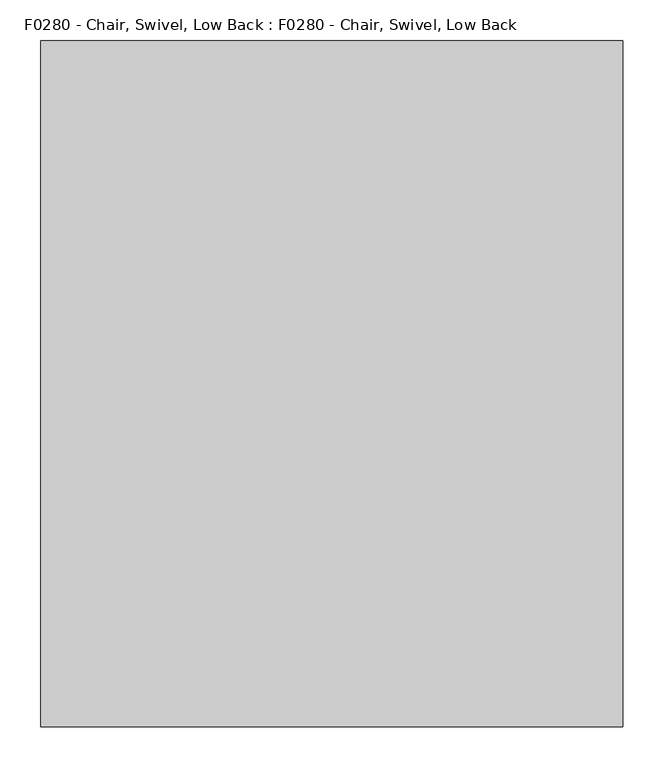
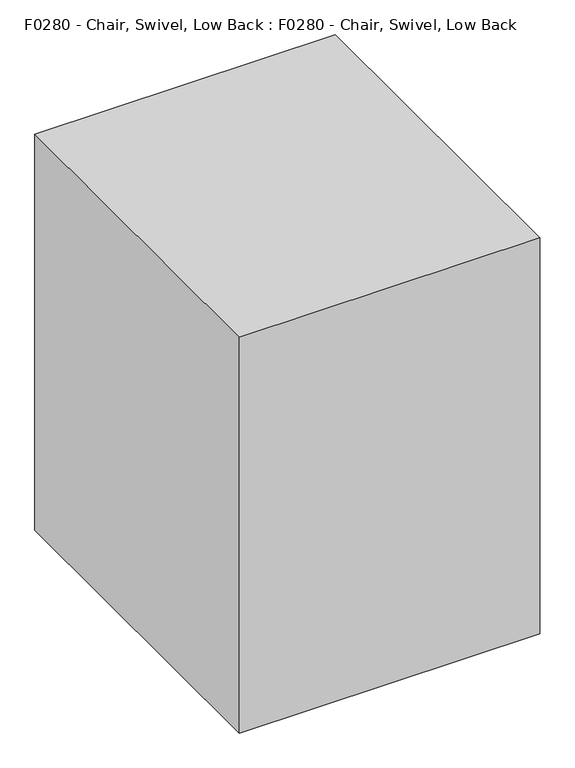
"""IFC4 building model written with IfcOpenShell, lengths in millimetres: proxy geometry, F0280 - Chair, Swivel, Low Back : F0280 - Chair, Swivel, Low Back."""

import ifcopenshell
import ifcopenshell.guid

model = None  # the IFC model being written
_history = None  # IfcOwnerHistory: only IFC2X3 demands one
_inside = {}  # id of a spatial element -> (the spatial element, [elements in it])
_under = {}  # id of a project, library or spatial element -> (it, [spatial elements below it])
_declared = {}  # id of a project -> (the project, [libraries it declares])
_typed = {}  # id of a type object -> (the type object, [elements of that type])
_made_of = {}  # id of a material, layer set ... -> (it, [elements and type objects made of it])


def new_model(schema):
    """Start an empty IFC model of exactly this schema.

    Asked for "IFC4X3", IfcOpenShell would pick the latest addendum, in which some entities
    have other attributes; the version numbers below select the first issue.
    IFC2X3 requires an IfcOwnerHistory on every rooted entity: one is made here for all.
    """
    global model, _history
    if schema == "IFC4X3":
        model = ifcopenshell.file(schema_version=(4, 3, 0, 0))
    else:
        model = ifcopenshell.file(schema=schema)
    _inside.clear()
    _under.clear()
    _declared.clear()
    _typed.clear()
    _made_of.clear()
    _history = None
    if model.schema == "IFC2X3":
        org = make("IfcOrganization", Name="unknown")
        user = make(
            "IfcPersonAndOrganization",
            ThePerson=make("IfcPerson", FamilyName="unknown"),
            TheOrganization=org,
        )
        app = make(
            "IfcApplication",
            ApplicationDeveloper=org,
            Version="unknown",
            ApplicationFullName="unknown",
            ApplicationIdentifier="unknown",
        )
        _history = make(
            "IfcOwnerHistory",
            OwningUser=user,
            OwningApplication=app,
            ChangeAction="ADDED",
            CreationDate=0,
        )
    return model


def make(cls, **values):
    """One entity of the class cls with the attributes given. An attribute that is None is left unset."""
    return model.create_entity(
        cls, **{name: value for name, value in values.items() if value is not None}
    )


def rooted(cls, **values):
    """An entity with a GlobalId (a new one), such as an element, a storey or a relation."""
    return make(cls, GlobalId=ifcopenshell.guid.new(), OwnerHistory=_history, **values)


def si_unit(unit_type, name, prefix=None):
    """IfcSIUnit, for example si_unit("LENGTHUNIT", "METRE", prefix="MILLI")."""
    return make("IfcSIUnit", UnitType=unit_type, Prefix=prefix, Name=name)


def assignment(units):
    """IfcUnitAssignment: the units of a project."""
    return None if units is None else make("IfcUnitAssignment", Units=units)


def point(xyz):
    """IfcCartesianPoint."""
    return None if xyz is None else make("IfcCartesianPoint", Coordinates=xyz)


def direction(xyz):
    """IfcDirection."""
    return None if xyz is None else make("IfcDirection", DirectionRatios=xyz)


def frame(location, z_axis=None, x_axis=None):
    """IfcAxis2Placement3D, a coordinate frame: its origin and axes. An axis left out is left unset."""
    return make(
        "IfcAxis2Placement3D",
        Location=point(location),
        Axis=direction(z_axis),
        RefDirection=direction(x_axis),
    )


def frame_2d(location, x_axis=None):
    """IfcAxis2Placement2D, a coordinate frame in the plane: its origin and x axis."""
    return make(
        "IfcAxis2Placement2D", Location=point(location), RefDirection=direction(x_axis)
    )


def origin():
    """The frame at (0, 0, 0) with its axes left unset."""
    return frame((0.0, 0.0, 0.0))


def origin_with_axes():
    """The frame at (0, 0, 0) with the z axis (0, 0, 1) and the x axis (1, 0, 0) written out."""
    return frame((0.0, 0.0, 0.0), z_axis=(0.0, 0.0, 1.0), x_axis=(1.0, 0.0, 0.0))


def origin_2d():
    """The frame at (0, 0) in the plane with its x axis left unset."""
    return frame_2d((0.0, 0.0))


def place(relative_to, where):
    """IfcLocalPlacement: puts the frame where relative to a parent placement (None: the world)."""
    return make(
        "IfcLocalPlacement", PlacementRelTo=relative_to, RelativePlacement=where
    )


def context(
    kind, dimensions, precision=None, world=None, true_north=None, identifier=None
):
    """IfcGeometricRepresentationContext, for example the 3D "Model" context."""
    return make(
        "IfcGeometricRepresentationContext",
        ContextIdentifier=identifier,
        ContextType=kind,
        CoordinateSpaceDimension=dimensions,
        Precision=precision,
        WorldCoordinateSystem=world,
        TrueNorth=true_north,
    )


def project(units=None, contexts=None):
    """IfcProject with its units and contexts."""
    return rooted(
        "IfcProject",
        Name="project",
        RepresentationContexts=contexts,
        UnitsInContext=assignment(units),
    )


def spatial(cls, under=None, at=None, **own):
    """A site, building, storey or space (cls), placed at a placement, below another one or the project."""
    s = rooted(cls, ObjectPlacement=at, **own)
    if under is not None:
        _under.setdefault(under.id(), (under, []))[1].append(s)
    return s


def polyline(points):
    """IfcPolyline through the points."""
    return make("IfcPolyline", Points=[point(p) for p in points])


def circle_curve(where, radius):
    """IfcCircle in the frame where."""
    return make("IfcCircle", Position=where, Radius=radius)


def ellipse_curve(where, semi_axis1, semi_axis2):
    """IfcEllipse in the frame where."""
    return make(
        "IfcEllipse", Position=where, SemiAxis1=semi_axis1, SemiAxis2=semi_axis2
    )


def trimmed(basis, trim1, trim2, sense, master):
    """IfcTrimmedCurve: the piece of a basis curve between two trims."""
    return make(
        "IfcTrimmedCurve",
        BasisCurve=basis,
        Trim1=trim1,
        Trim2=trim2,
        SenseAgreement=sense,
        MasterRepresentation=master,
    )


def segment(curve, same_sense, transition):
    """IfcCompositeCurveSegment."""
    return make(
        "IfcCompositeCurveSegment",
        Transition=transition,
        SameSense=same_sense,
        ParentCurve=curve,
    )


def composite_curve(segments, self_intersect=None):
    """IfcCompositeCurve: segments joined end to end."""
    return make("IfcCompositeCurve", Segments=segments, SelfIntersect=self_intersect)


def outline(outer, holes=None, kind="AREA"):
    """IfcArbitraryClosedProfileDef: a profile drawn as a closed curve; with holes, ...WithVoids."""
    if holes is None:
        return make("IfcArbitraryClosedProfileDef", ProfileType=kind, OuterCurve=outer)
    return make(
        "IfcArbitraryProfileDefWithVoids",
        ProfileType=kind,
        OuterCurve=outer,
        InnerCurves=holes,
    )


def extrude(swept, where, along, depth):
    """IfcExtrudedAreaSolid: the profile swept, set in the frame where, extruded along a direction by depth."""
    return make(
        "IfcExtrudedAreaSolid",
        SweptArea=swept,
        Position=where,
        ExtrudedDirection=direction(along),
        Depth=depth,
    )


def shape(context_of_items, identifier, shape_type, items):
    """IfcShapeRepresentation: the items that make up one representation, for example the "Body"."""
    return make(
        "IfcShapeRepresentation",
        ContextOfItems=context_of_items,
        RepresentationIdentifier=identifier,
        RepresentationType=shape_type,
        Items=items,
    )


def source(mapping_origin, context_of_items, identifier, shape_type, items):
    """IfcRepresentationMap: a shape defined once, which mapped items show again and again."""
    return make(
        "IfcRepresentationMap",
        MappingOrigin=mapping_origin,
        MappedRepresentation=shape(context_of_items, identifier, shape_type, items),
    )


def transform(
    local_origin,
    x_axis=None,
    y_axis=None,
    z_axis=None,
    scale=None,
    scale2=None,
    scale3=None,
    uniform=True,
):
    """IfcCartesianTransformationOperator3D, or its non-uniform kind. x_axis, y_axis, z_axis: its Axis1, 2, 3."""
    if uniform:
        return make(
            "IfcCartesianTransformationOperator3D",
            Axis1=direction(x_axis),
            Axis2=direction(y_axis),
            LocalOrigin=point(local_origin),
            Scale=scale,
            Axis3=direction(z_axis),
        )
    return make(
        "IfcCartesianTransformationOperator3DnonUniform",
        Axis1=direction(x_axis),
        Axis2=direction(y_axis),
        LocalOrigin=point(local_origin),
        Scale=scale,
        Axis3=direction(z_axis),
        Scale2=scale2,
        Scale3=scale3,
    )


def mapped(mapping_source, mapping_target):
    """IfcMappedItem: shows the shape of a source again, moved by a transform."""
    return make(
        "IfcMappedItem", MappingSource=mapping_source, MappingTarget=mapping_target
    )


def made_of(thing, what):
    """Note that an element or type object is made of a material, layer set ...; save() writes the relation."""
    if what is not None:
        _made_of.setdefault(what.id(), (what, []))[1].append(thing)
    return thing


def element(
    cls,
    number,
    at=None,
    inside=None,
    cuts=None,
    type_object=None,
    material=None,
    context=None,
    identifier="Body",
    shape_type=None,
    held_by="IfcProductDefinitionShape",
    body=None,
    shapes=None,
    **own,
):
    """One element of the class cls, such as IfcWall. Its Tag is "e" and its number.

    at: its placement. inside: the storey or other place that contains it. cuts: it is an
    opening in that element (IfcRelVoidsElement). A single representation is given by context,
    identifier, shape_type and body (its items); several are given by shapes. held_by: the class
    of the entity that holds the representations. save() writes the other relations.
    """
    e = rooted(cls, Tag="e%d" % number, ObjectPlacement=at, **own)
    if body is not None:
        shapes = [shape(context, identifier, shape_type, body)]
    if shapes is not None:
        e.Representation = make(held_by, Representations=shapes)
    if inside is not None:
        _inside.setdefault(inside.id(), (inside, []))[1].append(e)
    if cuts is not None:
        rooted(
            "IfcRelVoidsElement", RelatingBuildingElement=cuts, RelatedOpeningElement=e
        )
    if type_object is not None:
        _typed.setdefault(type_object.id(), (type_object, []))[1].append(e)
    return made_of(e, material)


def aggregate(whole, parts):
    """IfcRelAggregates: a whole, such as a stair, and the parts it consists of."""
    return rooted("IfcRelAggregates", RelatingObject=whole, RelatedObjects=parts)


def save(model, path):
    """Write the relations noted so far, then the file.

    IfcRelAggregates (storeys below a building ...), IfcRelContainedInSpatialStructure (elements
    in a storey), IfcRelDefinesByType, IfcRelAssociatesMaterial and IfcRelDeclares: one each for
    every whole, place, type object, material and project.
    """
    for whole, parts in _under.values():
        aggregate(whole, parts)
    for where, things in _inside.values():
        rooted(
            "IfcRelContainedInSpatialStructure",
            RelatedElements=things,
            RelatingStructure=where,
        )
    for kind, things in _typed.values():
        rooted("IfcRelDefinesByType", RelatedObjects=things, RelatingType=kind)
    for what, things in _made_of.values():
        rooted("IfcRelAssociatesMaterial", RelatedObjects=things, RelatingMaterial=what)
    for by, libraries in _declared.values():
        rooted("IfcRelDeclares", RelatingContext=by, RelatedDefinitions=libraries)
    model.write(path)


def plane_surface(at):
    """IfcPlane: the flat surface through the origin of the frame at, square to its z axis."""
    return make("IfcPlane", Position=at)


def cylinder_surface(at, radius):
    """IfcCylindricalSurface: all points at the distance radius from the z axis of the frame at."""
    return make("IfcCylindricalSurface", Position=at, Radius=radius)


def revolved_surface(curve, axis_point, axis_direction):
    """IfcSurfaceOfRevolution: the curve turned about the line through axis_point along axis_direction."""
    return make(
        "IfcSurfaceOfRevolution",
        SweptCurve=make("IfcArbitraryOpenProfileDef", ProfileType="CURVE", Curve=curve),
        AxisPosition=make("IfcAxis1Placement", Location=point(axis_point), Axis=direction(axis_direction)),
    )


def advanced_brep(points, edges, surfaces, faces):
    """IfcAdvancedBrep: a solid bounded by faces that lie on surfaces and meet in shared edges.

    An edge is (start, end): straight between two places in points (the first is 0);
    or (start, end, curve); or (start, end, curve, False) where it runs against its curve.
    A face is (place in surfaces, loops), or (place, loops, False) where it looks against
    its surface's normal. A loop lists edges by number (the first is 1), with a minus sign
    where the edge is run from its end to its start. The first loop is the outer one.
    """
    corners = [point(p) for p in points]
    vertices = [make("IfcVertexPoint", VertexGeometry=c) for c in corners]
    made = []
    for start, end, *more in edges:
        made.append(
            make(
                "IfcEdgeCurve",
                EdgeStart=vertices[start],
                EdgeEnd=vertices[end],
                EdgeGeometry=more[0] if more else make("IfcPolyline", Points=[corners[start], corners[end]]),
                SameSense=more[1] if len(more) > 1 else True,
            )
        )
    hull = []
    for where, loops, *sense in faces:
        bounds = []
        for j, loop in enumerate(loops):
            ring = [make("IfcOrientedEdge", EdgeElement=made[abs(k) - 1], Orientation=k > 0) for k in loop]
            bounds.append(
                make(
                    "IfcFaceOuterBound" if j == 0 else "IfcFaceBound",
                    Bound=make("IfcEdgeLoop", EdgeList=ring),
                    Orientation=True,
                )
            )
        hull.append(make("IfcAdvancedFace", Bounds=bounds, FaceSurface=surfaces[where], SameSense=sense[0] if sense else True))
    return make("IfcAdvancedBrep", Outer=make("IfcClosedShell", CfsFaces=hull))


def f0280_chair_swivel_low_back_f0280_chair_swivel_low_back_fbc83231(model_context):
    return source(origin(), model_context, "Body", "SolidModel", [
        advanced_brep(
        [(20.5891067, -0.9088165, 158.3164474), (20.5891067, -0.9088165, 212.7487443), (12.606954, 16.2089653, 212.7487443), (12.606954, 16.2089653, 158.3164474), (283.7284885, 121.7950923, 57.6571213), (283.7284885, 121.7950923, 86.0096871), (287.501904, 133.9556376, 82.2734822), (275.3053581, 138.7072429, 86.2220806), (275.3053581, 138.7072429, 57.8258095), (287.501904, 133.9556376, 54.689734)],
        [
            (0, 1),
            (1, 2),
            (2, 3),
            (3, 0),
            (0, 4),
            (4, 5),
            (5, 1),
            (5, 6, ellipse_curve(frame((278.918781, 129.9532617, 86.4074773), z_axis=(0.3625792018206629, 0.16907345849670724, 0.9164881276039822), x_axis=(0.8306203267741233, 0.3873246193939933, -0.40006188516396646)), 10.333389, 9.4704283)),
            (6, 7, ellipse_curve(frame((278.918781, 129.9532617, 86.4074773), z_axis=(0.3625792018206629, 0.16907345849670724, 0.9164881276039822), x_axis=(0.8306203267741233, 0.3873246193939933, -0.40006188516396646)), 10.333389, 9.4704283)),
            (7, 2),
            (7, 8),
            (8, 3),
            (8, 9, ellipse_curve(frame((278.918781, 129.9532617, 57.9730562), z_axis=(-0.2968743688836678, -0.13843479172039067, -0.9448287768380342), x_axis=(0.8563056778646188, 0.3993018953098915, -0.3275646233321667)), 10.0234334, 9.4704283)),
            (9, 4, ellipse_curve(frame((278.918781, 129.9532617, 57.9730562), z_axis=(-0.2968743688836678, -0.13843479172039067, -0.9448287768380342), x_axis=(0.8563056778646188, 0.3993018953098915, -0.3275646233321667)), 10.0234334, 9.4704283)),
            (6, 9),
        ],
        [
            plane_surface(frame((16.5980304, 7.6500744, 185.5325958), z_axis=(-0.9063077870366449, -0.42261826174071043, 0.0), x_axis=(-0.42261826174071043, 0.9063077870366449, 0.0))),
            plane_surface(frame((20.5891067, -0.9088165, 185.5325958), z_axis=(0.4226182617407104, -0.9063077870366448, 0.0), x_axis=(0.0, 0.0, 1.0))),
            plane_surface(frame((16.5980304, 7.6500744, 212.7487443), z_axis=(0.36257920182066294, 0.16907345849670727, 0.9164881276039825), x_axis=(-0.42261826174071043, 0.9063077870366449, 0.0))),
            plane_surface(frame((12.606954, 16.2089653, 185.5325958), z_axis=(-0.4226182617407102, 0.906307787036645, 0.0), x_axis=(0.0, 0.0, -1.0))),
            plane_surface(frame((16.5980304, 7.6500744, 158.3164474), z_axis=(-0.29687436888366786, -0.1384347917203907, -0.9448287768380345), x_axis=(0.42261826174071043, -0.9063077870366449, 0.0))),
            cylinder_surface(frame((278.918781, 129.9532617, 0.0), z_axis=(0.0, 0.0, -1.0000000000000002), x_axis=(-0.9063077870366449, -0.42261826174071043, 0.0)), 9.4704283),
        ],
        [
            (0, [[1, 2, 3, 4]]),
            (1, [[5, 6, 7, -1]]),
            (2, [[-7, 8, 9, 10, -2]]),
            (3, [[-10, 11, 12, -3]]),
            (4, [[-12, 13, 14, -5, -4]]),
            (5, [[-13, -11, -9, 15]]),
            (5, [[-8, -6, -14, -15]]),
        ],
    ),
        extrude(outline(composite_curve([segment(trimmed(circle_curve(frame_2d((-0.4565328, -0.2009494)), 25.4), [point((24.9434672, -0.2009494))], [point((-25.8565328, -0.2009494))], False, "CARTESIAN"), True, "CONTINUOUS"), segment(trimmed(circle_curve(frame_2d((-0.4565328, -0.2009494)), 25.4), [point((-25.8565328, -0.2009494))], [point((24.9434672, -0.2009494))], False, "CARTESIAN"), True, "CONTINUOUS")], self_intersect=False)), frame((0.0, 0.0, 154.0271692), z_axis=(0.0, 0.0, 1.0), x_axis=(1.0, 0.0, 0.0)), (0.0, 0.0, 1.0), 58.7215752),
        advanced_brep(
        [(-229.5082147, 191.2947504, 328.6387079), (-229.5082147, 216.926585, 331.293346), (236.3508412, 215.7557493, 331.1720849), (232.0214447, 190.8605661, 328.5937403), (-229.5082147, 284.2177228, 855.6310718), (232.0214447, 283.8251028, 855.8218273), (236.3508412, 306.337077, 844.8843217), (-229.5082147, 307.3958289, 844.3699241)],
        [
            (0, 1, circle_curve(frame((-229.5082147, 204.1106677, 329.9660269), z_axis=(0.0, 0.10301698777210262, -0.9946795967699159), x_axis=(-1.0, 0.0, 0.0)), 12.8844679)),
            (1, 2, circle_curve(frame((0.0, -1130.5045098, 191.7425871), z_axis=(0.0, 0.10301698777210262, -0.9946795967699159), x_axis=(-1.0, 0.0, 0.0)), 1373.9428628)),
            (2, 3, circle_curve(frame((232.0214447, 203.6806144, 329.9214872), z_axis=(0.0, 0.10301698777210262, -0.9946795967699159), x_axis=(-1.0, 0.0, 0.0)), 12.888621)),
            (3, 0, circle_curve(frame((0.0, -1130.5045098, 191.7425871), z_axis=(0.0, -0.10301698777210262, 0.9946795967699159), x_axis=(-1.0, 0.0, 0.0)), 1348.5428628)),
            (4, 5, circle_curve(frame((0.0, -911.0460573, 1436.3533187), z_axis=(0.0, -0.4370047614753844, -0.8994591922082082), x_axis=(-1.0, 0.0, 0.0)), 1348.5428628)),
            (5, 6, circle_curve(frame((232.0214447, 295.4178914, 850.1894385), z_axis=(0.0, 0.4370047614753844, 0.8994591922082082), x_axis=(-1.0, 0.0, 0.0)), 12.888621)),
            (6, 7, circle_curve(frame((0.0, -911.0460573, 1436.3533187), z_axis=(0.0, 0.4370047614753844, 0.8994591922082082), x_axis=(-1.0, 0.0, 0.0)), 1373.9428628)),
            (7, 4, circle_curve(frame((-229.5082147, 295.8067759, 850.0004979), z_axis=(0.0, 0.4370047614753844, 0.8994591922082082), x_axis=(-1.0, 0.0, 0.0)), 12.8844679)),
            (4, 0, circle_curve(frame((-229.5082147, 1161.9751957, 429.1701512), z_axis=(1.0, 0.0, 0.0), x_axis=(0.0, -0.9946795967699159, -0.10301698777210261)), 975.8724803)),
            (3, 5, circle_curve(frame((232.0214447, 1161.9751957, 429.1701512), z_axis=(-1.0, 0.0, 0.0), x_axis=(0.0, -0.9946795967699159, -0.10301698777210261)), 976.308987)),
            (2, 6, circle_curve(frame((236.3508412, 1161.9751957, 429.1701512), z_axis=(-1.0, 0.0, 0.0), x_axis=(0.0, -0.9946795967699159, -0.10301698777210261)), 951.280643)),
            (1, 7, circle_curve(frame((-229.5082147, 1161.9751957, 429.1701512), z_axis=(-1.0, 0.0, 0.0), x_axis=(0.0, -0.9946795967699159, -0.10301698777210261)), 950.1035446)),
        ],
        [
            plane_surface(frame((-317.5, 173.1564347, 326.7601586), z_axis=(0.0, 0.10301698777210258, -0.994679596769916), x_axis=(-1.0, 0.0, 0.0))),
            plane_surface(frame((-317.5, 267.815783, 863.6), z_axis=(0.0, 0.4370047614753844, 0.8994591922082082), x_axis=(-1.0, 0.0, 0.0))),
            revolved_surface(trimmed(ellipse_curve(frame((0.0, -1130.5045098, 191.7425871), z_axis=(0.0, 0.10301698777210262, -0.9946795967699159), x_axis=(-1.0, 0.0, 0.0)), 1348.5428628, 1348.5428628), [point((-229.5082147, 191.2947504, 328.6387079))], [point((232.0214447, 190.8605661, 328.5937403))], True, "CARTESIAN"), (-317.5, 1161.9751957, 429.1701512), (1.0, 0.0, 0.0)),
            revolved_surface(trimmed(ellipse_curve(frame((232.0214447, 203.6806144, 329.9214872), z_axis=(0.0, -0.10301698777210262, 0.9946795967699159), x_axis=(-1.0, 0.0, 0.0)), 12.888621, 12.888621), [point((232.0214447, 190.8605661, 328.5937403))], [point((236.3508412, 215.7557493, 331.1720849))], True, "CARTESIAN"), (-317.5, 1161.9751957, 429.1701512), (1.0, 0.0, 0.0)),
            revolved_surface(trimmed(ellipse_curve(frame((0.0, -1130.5045098, 191.7425871), z_axis=(0.0, -0.10301698777210262, 0.9946795967699159), x_axis=(-1.0, 0.0, 0.0)), 1373.9428628, 1373.9428628), [point((236.3508412, 215.7557493, 331.1720849))], [point((-229.5082147, 216.926585, 331.293346))], True, "CARTESIAN"), (-317.5, 1161.9751957, 429.1701512), (1.0, 0.0, 0.0)),
            revolved_surface(trimmed(ellipse_curve(frame((-229.5082147, 204.1106677, 329.9660269), z_axis=(0.0, -0.10301698777210262, 0.9946795967699159), x_axis=(-1.0, 0.0, 0.0)), 12.8844679, 12.8844679), [point((-229.5082147, 216.926585, 331.293346))], [point((-229.5082147, 191.2947504, 328.6387079))], True, "CARTESIAN"), (-317.5, 1161.9751957, 429.1701512), (1.0, 0.0, 0.0)),
        ],
        [
            (0, [[1, 2, 3, 4]]),
            (1, [[5, 6, 7, 8]]),
            (2, [[-5, 9, -4, 10]]),
            (3, [[-6, -10, -3, 11]]),
            (4, [[-7, -11, -2, 12]]),
            (5, [[-8, -12, -1, -9]]),
        ],
    ),
        extrude(outline(composite_curve([segment(polyline([(-213.079753, 174.0379297), (221.4112726, 174.0379297), (221.4112726, -182.9075832)]), True, "CONTINUOUS"), segment(trimmed(circle_curve(frame_2d((194.6657598, -182.9075832)), 26.7455128), [point((221.4112726, -182.9075832))], [point((194.6657598, -209.653096))], False, "CARTESIAN"), True, "CONTINUOUS"), segment(polyline([(194.6657598, -209.653096), (-186.3342402, -209.653096)]), True, "CONTINUOUS"), segment(trimmed(circle_curve(frame_2d((-186.3342402, -182.9075832)), 26.7455128), [point((-186.3342402, -209.653096))], [point((-213.079753, -182.9075832))], False, "CARTESIAN"), True, "CONTINUOUS"), segment(polyline([(-213.079753, -182.9075832), (-213.079753, 174.0379297)]), True, "CONTINUOUS")], self_intersect=False)), frame((0.0, 0.0, 324.0440254), z_axis=(0.0, 0.0, 1.0), x_axis=(1.0, 0.0, 0.0)), (0.0, 0.0, 1.0), 67.8491407),
        advanced_brep(
        [(-213.079753, 172.6924168, 391.8931661), (-213.079753, 172.6924168, 324.0440254), (-211.7342402, 174.0379297, 324.0440254), (-211.7342402, 174.0379297, 391.8931661), (-213.079753, -182.9075832, 391.8931661), (-213.079753, -182.9075832, 324.0440254), (-186.3342402, -209.653096, 391.8931661), (-186.3342402, -209.653096, 324.0440254), (194.6657598, -209.653096, 391.8931661), (194.6657598, -209.653096, 324.0440254), (221.4112726, -182.9075832, 391.8931661), (221.4112726, -182.9075832, 324.0440254), (221.4112726, 172.6924168, 391.8931661), (221.4112726, 172.6924168, 324.0440254), (220.0657598, 174.0379297, 391.8931661), (220.0657598, 174.0379297, 324.0440254)],
        [
            (0, 1),
            (1, 2, circle_curve(frame((-211.7342402, 172.6924168, 324.0440254), z_axis=(0.0, 0.0, -1.0), x_axis=(0.0, 1.0, 0.0)), 1.3455128)),
            (2, 3),
            (3, 0, circle_curve(frame((-211.7342402, 172.6924168, 391.8931661), z_axis=(0.0, 0.0, 1.0), x_axis=(0.0, 1.0, 0.0)), 1.3455128)),
            (1, 0, circle_curve(frame((-213.079753, 172.6924168, 357.9685958), z_axis=(0.0, 1.0, 0.0), x_axis=(1.0, 0.0, 0.0)), 33.9245703)),
            (3, 2, circle_curve(frame((-211.7342402, 174.0379297, 357.9685958), z_axis=(-1.0, 0.0, 0.0), x_axis=(0.0, -1.0, 0.0)), 33.9245703)),
            (0, 4),
            (4, 5),
            (5, 1),
            (5, 4, circle_curve(frame((-213.079753, -182.9075832, 357.9685958), z_axis=(0.0, 1.0, 0.0), x_axis=(1.0, 0.0, 0.0)), 33.9245703)),
            (6, 7),
            (7, 5, circle_curve(frame((-186.3342402, -182.9075832, 324.0440254), z_axis=(0.0, 0.0, -1.0), x_axis=(-1.0, 0.0, 0.0)), 26.7455128)),
            (4, 6, circle_curve(frame((-186.3342402, -182.9075832, 391.8931661), z_axis=(0.0, 0.0, 1.0), x_axis=(-1.0, 0.0, 0.0)), 26.7455128)),
            (7, 6, circle_curve(frame((-186.3342402, -209.653096, 357.9685958), z_axis=(-1.0, 0.0, 0.0), x_axis=(0.0, 1.0, 0.0)), 33.9245703)),
            (6, 8),
            (8, 9),
            (9, 7),
            (9, 8, circle_curve(frame((194.6657598, -209.653096, 357.9685958), z_axis=(-1.0, 0.0, 0.0), x_axis=(0.0, 1.0, 0.0)), 33.9245703)),
            (10, 11),
            (11, 9, circle_curve(frame((194.6657598, -182.9075832, 324.0440254), z_axis=(0.0, 0.0, -1.0), x_axis=(0.0, -1.0, 0.0)), 26.7455128)),
            (8, 10, circle_curve(frame((194.6657598, -182.9075832, 391.8931661), z_axis=(0.0, 0.0, 1.0), x_axis=(0.0, -1.0, 0.0)), 26.7455128)),
            (11, 10, circle_curve(frame((221.4112726, -182.9075832, 357.9685958), z_axis=(0.0, -1.0, 0.0), x_axis=(-1.0, 0.0, 0.0)), 33.9245703)),
            (10, 12),
            (12, 13),
            (13, 11),
            (13, 12, circle_curve(frame((221.4112726, 172.6924168, 357.9685958), z_axis=(0.0, -1.0, 0.0), x_axis=(-1.0, 0.0, 0.0)), 33.9245703)),
            (14, 15),
            (15, 13, circle_curve(frame((220.0657598, 172.6924168, 324.0440254), z_axis=(0.0, 0.0, -1.0), x_axis=(1.0, 0.0, 0.0)), 1.3455128)),
            (12, 14, circle_curve(frame((220.0657598, 172.6924168, 391.8931661), z_axis=(0.0, 0.0, 1.0), x_axis=(1.0, 0.0, 0.0)), 1.3455128)),
            (15, 14, circle_curve(frame((220.0657598, 174.0379297, 357.9685958), z_axis=(1.0, 0.0, 0.0), x_axis=(0.0, -1.0, 0.0)), 33.9245703)),
            (14, 3),
            (2, 15),
        ],
        [
            revolved_surface(polyline([(-211.7342402, 174.03792959999998, 324.0440254), (-211.7342402, 174.03792959999998, 391.8931661)]), (-211.7342402, 172.6924168, 0.0), (0.0, 0.0, -1.0)),
            revolved_surface(trimmed(ellipse_curve(frame((-211.7342402, 174.0379297, 357.9685958), z_axis=(-1.0, 0.0, 0.0), x_axis=(0.0, -1.0, 0.0)), 33.9245703, 33.9245703), [point((-211.7342402, 174.0379297, 391.8931661))], [point((-211.7342402, 174.0379297, 324.0440254))], True, "CARTESIAN"), (-211.7342402, 172.6924168, 0.0), (0.0, 0.0, -1.0)),
            plane_surface(frame((-213.079753, 172.6924168, 324.0440254), z_axis=(1.0, 0.0, 0.0), x_axis=(0.0, -1.0, 0.0))),
            cylinder_surface(frame((-213.079753, 172.6924168, 357.9685958), z_axis=(0.0, 1.0, 0.0), x_axis=(1.0, 0.0, 0.0)), 33.9245703),
            revolved_surface(polyline([(-213.079753, -182.9075832, 324.0440254), (-213.079753, -182.9075832, 391.8931661)]), (-186.3342402, -182.9075832, 0.0), (0.0, 0.0, -1.0)),
            revolved_surface(trimmed(ellipse_curve(frame((-213.079753, -182.9075832, 357.9685958), z_axis=(0.0, -1.0, 0.0), x_axis=(1.0, 0.0, 0.0)), 33.9245703, 33.9245703), [point((-213.079753, -182.9075832, 391.8931661))], [point((-213.079753, -182.9075832, 324.0440254))], True, "CARTESIAN"), (-186.3342402, -182.9075832, 0.0), (0.0, 0.0, -1.0)),
            plane_surface(frame((-186.3342402, -209.653096, 324.0440254), z_axis=(0.0, 1.0, 0.0), x_axis=(1.0, 0.0, 0.0))),
            cylinder_surface(frame((-186.3342402, -209.653096, 357.9685958), z_axis=(-1.0, 0.0, 0.0), x_axis=(0.0, 1.0, 0.0)), 33.9245703),
            revolved_surface(polyline([(194.6657598, -209.653096, 324.0440254), (194.6657598, -209.653096, 391.8931661)]), (194.6657598, -182.9075832, 0.0), (0.0, 0.0, -1.0)),
            revolved_surface(trimmed(ellipse_curve(frame((194.6657598, -209.653096, 357.9685958), z_axis=(1.0, 0.0, 0.0), x_axis=(0.0, 1.0, 0.0)), 33.9245703, 33.9245703), [point((194.6657598, -209.653096, 391.8931661))], [point((194.6657598, -209.653096, 324.0440254))], True, "CARTESIAN"), (194.6657598, -182.9075832, 0.0), (0.0, 0.0, -1.0)),
            plane_surface(frame((221.4112726, -182.9075832, 324.0440254), z_axis=(-1.0, 0.0, 0.0), x_axis=(0.0, 1.0, 0.0))),
            cylinder_surface(frame((221.4112726, -182.9075832, 357.9685958), z_axis=(0.0, -1.0, 0.0), x_axis=(-1.0, 0.0, 0.0)), 33.9245703),
            revolved_surface(polyline([(221.4112726, 172.6924168, 324.0440254), (221.4112726, 172.6924168, 391.8931661)]), (220.0657598, 172.6924168, 0.0), (0.0, 0.0, -1.0)),
            revolved_surface(trimmed(ellipse_curve(frame((221.4112726, 172.6924168, 357.9685958), z_axis=(0.0, 1.0, 0.0), x_axis=(-1.0, 0.0, 0.0)), 33.9245703, 33.9245703), [point((221.4112726, 172.6924168, 391.8931661))], [point((221.4112726, 172.6924168, 324.0440254))], True, "CARTESIAN"), (220.0657598, 172.6924168, 0.0), (0.0, 0.0, -1.0)),
            plane_surface(frame((220.0657598, 174.0379297, 324.0440254), z_axis=(0.0, -1.0, 0.0), x_axis=(-1.0, 0.0, 0.0))),
            cylinder_surface(frame((220.0657598, 174.0379297, 357.9685958), z_axis=(1.0, 0.0, 0.0), x_axis=(0.0, -1.0, 0.0)), 33.9245703),
        ],
        [
            (0, [[1, 2, 3, 4]]),
            (1, [[5, -4, 6, -2]]),
            (2, [[7, 8, 9, -1]]),
            (3, [[-9, 10, -7, -5]]),
            (4, [[11, 12, -8, 13]]),
            (5, [[14, -13, -10, -12]]),
            (6, [[15, 16, 17, -11]]),
            (7, [[-17, 18, -15, -14]]),
            (8, [[19, 20, -16, 21]]),
            (9, [[22, -21, -18, -20]]),
            (10, [[23, 24, 25, -19]]),
            (11, [[-25, 26, -23, -22]]),
            (12, [[27, 28, -24, 29]]),
            (13, [[30, -29, -26, -28]]),
            (14, [[31, -3, 32, -27]]),
            (15, [[-32, -6, -31, -30]]),
        ],
    ),
        extrude(outline(composite_curve([segment(trimmed(circle_curve(origin_2d(), 12.7), [point((12.7, 0.0))], [point((-12.7, 0.0))], False, "CARTESIAN"), True, "CONTINUOUS"), segment(trimmed(circle_curve(origin_2d(), 12.7), [point((-12.7, 0.0))], [point((12.7, 0.0))], False, "CARTESIAN"), True, "CONTINUOUS")], self_intersect=False)), frame((0.0, 0.0, 212.7487443), z_axis=(0.0, 0.0, 1.0), x_axis=(1.0, 0.0, 0.0)), (0.0, 0.0, 1.0), 66.217703),
        extrude(outline(polyline([(355.6, -419.1), (-355.6, -419.1), (-355.6, 419.1), (355.6, 419.1), (355.6, -419.1)])), origin_with_axes(), (0.0, 0.0, 1.0), 990.6),
    ])


if __name__ == "__main__":
    model = new_model("IFC4")
    model_context = context("Model", 3, world=origin())
    ifc_project = project(units=[si_unit("LENGTHUNIT", "METRE", prefix="MILLI")], contexts=[model_context])
    site = spatial("IfcSite", under=ifc_project)
    building = spatial("IfcBuilding", under=site)
    placement = place(None, origin())
    f0280_chair_swivel_low_back_f0280_chair_swivel_low_back_shape = f0280_chair_swivel_low_back_f0280_chair_swivel_low_back_fbc83231(model_context)
    element("IfcBuildingElementProxy", 1, Name="F0280 - Chair, Swivel, Low Back : F0280 - Chair, Swivel, Low Back", ObjectType="F0280 - Chair, Swivel, Low Back : F0280 - Chair, Swivel, Low Back", at=placement, inside=building, context=model_context, shape_type="MappedRepresentation", body=[
        mapped(f0280_chair_swivel_low_back_f0280_chair_swivel_low_back_shape, transform((0.0, 0.0, 0.0), x_axis=(1.0, 0.0, 0.0), y_axis=(0.0, 1.0, 0.0), z_axis=(0.0, 0.0, 1.0))),
    ])
    save(model, "model.ifc")

# Revit data of these elements
# Type "F0280 - Chair, Swivel, Low Back : F0280 - Chair, Swivel, Low Back"
#   Watts2 = "0"
#   Watts1 = "0"
#   Unit_Issue = "EA"
#   UTIL_6_Misc = "-"
#   UTIL_5_NonMedGas = "-"
#   UTIL_4_MiscGas = "-"
#   UTIL_3_MedGas = "-"
#   UTIL_2_Elec = "-"
#   UTIL_1_WaterDrain = "-"
#   Nomenclature = "Chair, Swivel, Low Back"
#   NSN = "7110"
#   Location [instance default] = ""
#   JSN = "F0280"
#   Fund_Source_VA = "-"
#   Fund_Source_Navy = "-"
#   Fund_Source_Army = "-"
#   Fund_Source_AF = "-"
#   ELEC_Volts2 = "0"
#   ELEC_Volts1 = "0"
#   ELEC_Phase2 = "0"
#   ELEC_Phase1 = "0"
#   ELEC_HertzSwitch = "0"
#   ELEC_HertzDependent = "0"
#   ELEC_Hertz = "0"
#   ELEC_Amps2 = "0"
#   ELEC_Amps1 = "0"
#   DetailDescription = "Low back contemporary swivel chair, 37\" high X 25\" wide X 31\" deep with a five (5) caster swivel base, arms and foam padded seat and back upholstered with either woven textile fabric or vinyl."
#   CAT_VA = "C"
#   CAT_Navy = "C"
#   CAT_IHS = "-"
#   CAT_Army = "C"
#   CAT_AF = "C"
#   BTUperhour = "0"
#   Weight_IP = 49
#   DIM_Width_IP = 2' - 4"
#   DIM_Height_IP = 3' - 3"
#   DIM_Depth_IP = 2' - 9"
#   Assembly Code = ""
# Element 1 (IfcBuildingElementProxy, "F0280 - Chair, Swivel, Low Back : F0280 - Chair, Swivel, Low Back")
#   Location = "DUTY1"
#   Materials on its faces: "00 - bernhardt blitz - base", "00 - bernhardt blitz - Seat Fabric", "00 - bernhardt blitz - wheels", "00 - bernhardt blitz - arms", "00 - bernhardt blitz - mechanic", "00 - bernhardt blitz - Back Fabric", "EquipSpace"
# Materials
#   "00 - bernhardt blitz - base": class "Miscellaneous", colour RGB 192 192 192, transparency 0
#   "00 - bernhardt blitz - Seat Fabric": class "Miscellaneous", colour RGB 188 173 117, transparency 0
#   "00 - bernhardt blitz - wheels": class "Miscellaneous", colour RGB 51 51 51, transparency 0
#   "00 - bernhardt blitz - arms": class "Miscellaneous", colour RGB 51 51 51, transparency 0
#   "00 - bernhardt blitz - mechanic": class "Miscellaneous", colour RGB 62 62 62, transparency 0
#   "00 - bernhardt blitz - Back Fabric": class "Miscellaneous", colour RGB 93 93 93, transparency 0
#   "EquipSpace": class "Unassigned", colour RGB 221 217 195, transparency 0.5
